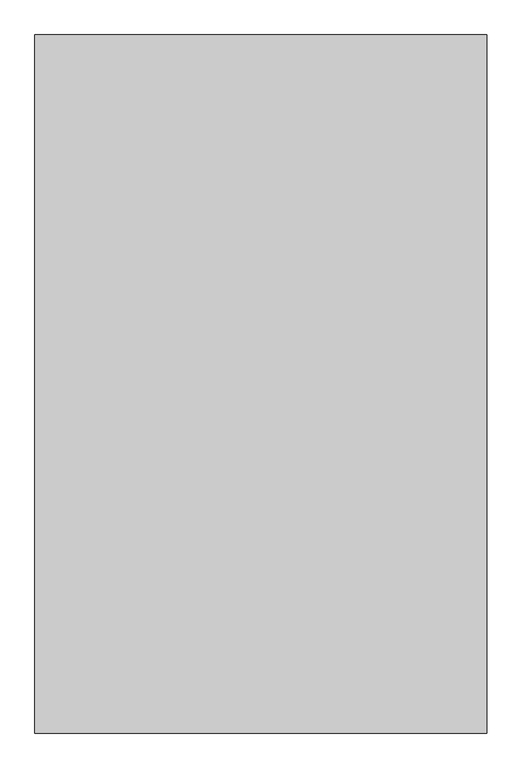
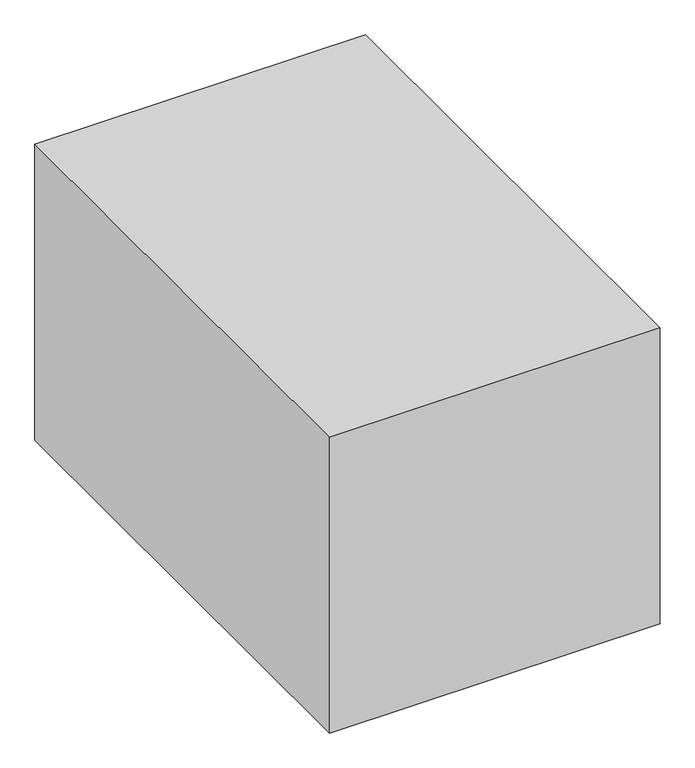
"""IFC4 building model written with IfcOpenShell, lengths in millimetres: proxy geometry, Space Planning Box_hec : Space Planning Box_hec."""

from ifc_helpers import new_model, si_unit, origin, origin_with_axes, place, context, project, spatial, polyline, outline, extrude, source, transform, mapped, element, save


def generic_models_d0c3260c(model_context):
    return source(origin(), model_context, "Body", "SweptSolid", [
        extrude(outline(polyline([(2750.0, 4250.0), (2750.0, -4250.0), (-2750.0, -4250.0), (-2750.0, 4250.0), (2750.0, 4250.0)])), origin_with_axes(), (0.0, 0.0, 1.0), 5200.0),
    ])


if __name__ == "__main__":
    model = new_model("IFC4")
    model_context = context("Model", 3, world=origin())
    ifc_project = project(units=[si_unit("LENGTHUNIT", "METRE", prefix="MILLI")], contexts=[model_context])
    site = spatial("IfcSite", under=ifc_project)
    building = spatial("IfcBuilding", under=site)
    placement = place(None, origin())
    generic_models_shape = generic_models_d0c3260c(model_context)
    element("IfcBuildingElementProxy", 1, Name="Space Planning Box_hec : Space Planning Box_hec", ObjectType="Space Planning Box_hec : Space Planning Box_hec", at=placement, inside=building, context=model_context, shape_type="MappedRepresentation", body=[
        mapped(generic_models_shape, transform((0.0, 0.0, 0.0), x_axis=(1.0, 0.0, 0.0), y_axis=(0.0, 1.0, 0.0), z_axis=(0.0, 0.0, 1.0))),
    ])
    save(model, "model.ifc")

# Revit data of these elements
# Type "Space Planning Box_hec : Space Planning Box_hec"
#   Type Comments = "..."
#   Room Name [instance default] = "?"
#   Interior Finish [instance default] = ""
#   Exterior Finish [instance default] = ""
#   Department [instance default] = ""
#   Assembly Code = "..."
#   ceiling height [instance default] = 0
#   Width [instance default] = 1524 mm
#   Program Area [instance default] = 0.00 m²
#   Length [instance default] = 1524 mm
#   Height [instance default] = 1524 mm
#   Area [instance default] = 2.32258 m²
#   Fill Color [instance default] = Cyan
#   Default Elevation = 0
# Element 1 (IfcBuildingElementProxy, "Space Planning Box_hec : Space Planning Box_hec")
#   Room Name = "Communication Room"
#   Interior Finish = "IW1..N/A,,WB2..N/A,,FL7..N/A,,CL4..N/A"
#   Exterior Finish = "N/A..N/A,,EW1..N/A"
#   Department = "CI"
#   ceiling height = 2700
#   Width = 5500 mm
#   Program Area = 46.75 m²
#   Length = 8500 mm
#   Height = 5200 mm
#   Area = 46.75 m²
#   Fill Color = Yellow
#   Materials on its faces: "Yellow"
# Materials
#   "Cyan": class "Generic", colour RGB 0 255 255, transparency 0.2, Cost = 0
#   "Yellow": class "Generic", colour RGB 255 255 0, transparency 0.2, Cost = 0
